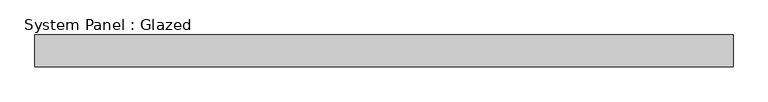
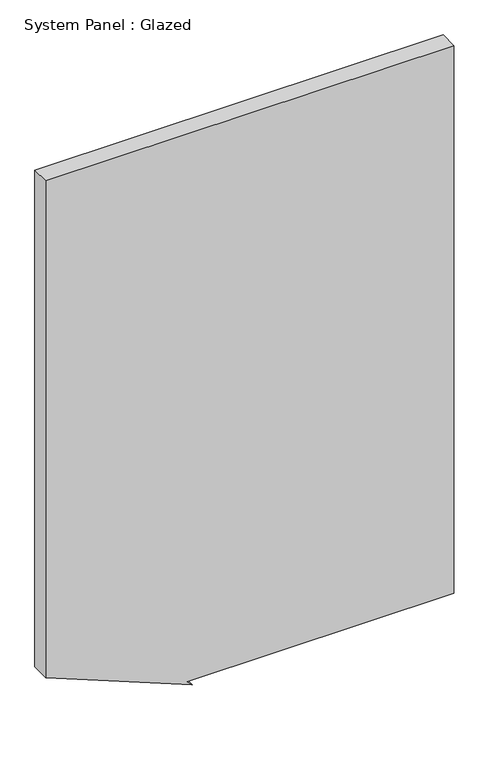
"""IFC4 building model written with IfcOpenShell, lengths in millimetres: plate geometry, System Panel : Glazed."""

from ifc_helpers import new_model, si_unit, frame, origin, place, context, project, spatial, polyline, outline, extrude, source, transform, mapped, element, save


def system_panel_glazed_6e92f89b(model_context):
    return source(origin(), model_context, "Body", "SweptSolid", [
        extrude(outline(polyline([(0.0, -155.080733), (12.8609324, -169.93636), (12.8609324, 550.0), (1572.8609324, 550.0), (1572.8609324, -550.0), (157.9677068, -550.0), (0.0, -155.080733)])), frame((0.0, -25.0, 0.0), z_axis=(0.0, 1.0, 0.0), x_axis=(0.0, 0.0, 1.0)), (0.0, 0.0, 1.0), 50.0),
    ])


if __name__ == "__main__":
    model = new_model("IFC4")
    model_context = context("Model", 3, world=origin())
    ifc_project = project(units=[si_unit("LENGTHUNIT", "METRE", prefix="MILLI")], contexts=[model_context])
    site = spatial("IfcSite", under=ifc_project)
    building = spatial("IfcBuilding", under=site)
    placement = place(None, origin())
    system_panel_glazed_shape = system_panel_glazed_6e92f89b(model_context)
    element("IfcPlate", 1, ObjectType="System Panel : Glazed", at=placement, inside=building, context=model_context, shape_type="MappedRepresentation", body=[
        mapped(system_panel_glazed_shape, transform((0.0, 0.0, 0.0), x_axis=(1.0, 0.0, 0.0), y_axis=(0.0, 1.0, 0.0), z_axis=(0.0, 0.0, 1.0))),
    ])
    save(model, "model.ifc")

# Revit data of these elements
# Type "System Panel : Glazed"
#   Type Mark = "CW-GLASS"
# Element 1 (IfcPlate, "System Panel : Glazed")
#   Materials on its faces: "Glass_Clear"
# Materials
#   "Glass_Clear": class "Glass", colour RGB 128 128 255, transparency 0.8, Comments = "Rendering appearance not upgraded ", Cost = 0
